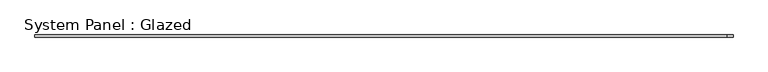
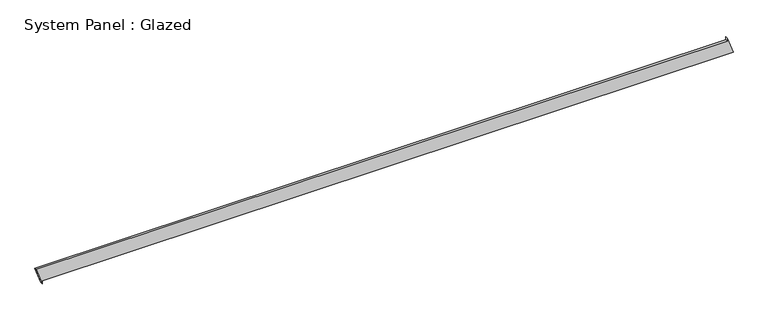
"""IFC4 building model written with IfcOpenShell, lengths in millimetres: plate geometry, System Panel : Glazed."""

import ifcopenshell
import ifcopenshell.guid

model = None  # the IFC model being written
_history = None  # IfcOwnerHistory: only IFC2X3 demands one
_inside = {}  # id of a spatial element -> (the spatial element, [elements in it])
_under = {}  # id of a project, library or spatial element -> (it, [spatial elements below it])
_declared = {}  # id of a project -> (the project, [libraries it declares])
_typed = {}  # id of a type object -> (the type object, [elements of that type])
_made_of = {}  # id of a material, layer set ... -> (it, [elements and type objects made of it])


def new_model(schema):
    """Start an empty IFC model of exactly this schema.

    Asked for "IFC4X3", IfcOpenShell would pick the latest addendum, in which some entities
    have other attributes; the version numbers below select the first issue.
    IFC2X3 requires an IfcOwnerHistory on every rooted entity: one is made here for all.
    """
    global model, _history
    if schema == "IFC4X3":
        model = ifcopenshell.file(schema_version=(4, 3, 0, 0))
    else:
        model = ifcopenshell.file(schema=schema)
    _inside.clear()
    _under.clear()
    _declared.clear()
    _typed.clear()
    _made_of.clear()
    _history = None
    if model.schema == "IFC2X3":
        org = make("IfcOrganization", Name="unknown")
        user = make(
            "IfcPersonAndOrganization",
            ThePerson=make("IfcPerson", FamilyName="unknown"),
            TheOrganization=org,
        )
        app = make(
            "IfcApplication",
            ApplicationDeveloper=org,
            Version="unknown",
            ApplicationFullName="unknown",
            ApplicationIdentifier="unknown",
        )
        _history = make(
            "IfcOwnerHistory",
            OwningUser=user,
            OwningApplication=app,
            ChangeAction="ADDED",
            CreationDate=0,
        )
    return model


def make(cls, **values):
    """One entity of the class cls with the attributes given. An attribute that is None is left unset."""
    return model.create_entity(
        cls, **{name: value for name, value in values.items() if value is not None}
    )


def rooted(cls, **values):
    """An entity with a GlobalId (a new one), such as an element, a storey or a relation."""
    return make(cls, GlobalId=ifcopenshell.guid.new(), OwnerHistory=_history, **values)


def si_unit(unit_type, name, prefix=None):
    """IfcSIUnit, for example si_unit("LENGTHUNIT", "METRE", prefix="MILLI")."""
    return make("IfcSIUnit", UnitType=unit_type, Prefix=prefix, Name=name)


def assignment(units):
    """IfcUnitAssignment: the units of a project."""
    return None if units is None else make("IfcUnitAssignment", Units=units)


def point(xyz):
    """IfcCartesianPoint."""
    return None if xyz is None else make("IfcCartesianPoint", Coordinates=xyz)


def direction(xyz):
    """IfcDirection."""
    return None if xyz is None else make("IfcDirection", DirectionRatios=xyz)


def frame(location, z_axis=None, x_axis=None):
    """IfcAxis2Placement3D, a coordinate frame: its origin and axes. An axis left out is left unset."""
    return make(
        "IfcAxis2Placement3D",
        Location=point(location),
        Axis=direction(z_axis),
        RefDirection=direction(x_axis),
    )


def origin():
    """The frame at (0, 0, 0) with its axes left unset."""
    return frame((0.0, 0.0, 0.0))


def place(relative_to, where):
    """IfcLocalPlacement: puts the frame where relative to a parent placement (None: the world)."""
    return make(
        "IfcLocalPlacement", PlacementRelTo=relative_to, RelativePlacement=where
    )


def context(
    kind, dimensions, precision=None, world=None, true_north=None, identifier=None
):
    """IfcGeometricRepresentationContext, for example the 3D "Model" context."""
    return make(
        "IfcGeometricRepresentationContext",
        ContextIdentifier=identifier,
        ContextType=kind,
        CoordinateSpaceDimension=dimensions,
        Precision=precision,
        WorldCoordinateSystem=world,
        TrueNorth=true_north,
    )


def project(units=None, contexts=None):
    """IfcProject with its units and contexts."""
    return rooted(
        "IfcProject",
        Name="project",
        RepresentationContexts=contexts,
        UnitsInContext=assignment(units),
    )


def spatial(cls, under=None, at=None, **own):
    """A site, building, storey or space (cls), placed at a placement, below another one or the project."""
    s = rooted(cls, ObjectPlacement=at, **own)
    if under is not None:
        _under.setdefault(under.id(), (under, []))[1].append(s)
    return s


def polyline(points):
    """IfcPolyline through the points."""
    return make("IfcPolyline", Points=[point(p) for p in points])


def outline(outer, holes=None, kind="AREA"):
    """IfcArbitraryClosedProfileDef: a profile drawn as a closed curve; with holes, ...WithVoids."""
    if holes is None:
        return make("IfcArbitraryClosedProfileDef", ProfileType=kind, OuterCurve=outer)
    return make(
        "IfcArbitraryProfileDefWithVoids",
        ProfileType=kind,
        OuterCurve=outer,
        InnerCurves=holes,
    )


def extrude(swept, where, along, depth):
    """IfcExtrudedAreaSolid: the profile swept, set in the frame where, extruded along a direction by depth."""
    return make(
        "IfcExtrudedAreaSolid",
        SweptArea=swept,
        Position=where,
        ExtrudedDirection=direction(along),
        Depth=depth,
    )


def shape(context_of_items, identifier, shape_type, items):
    """IfcShapeRepresentation: the items that make up one representation, for example the "Body"."""
    return make(
        "IfcShapeRepresentation",
        ContextOfItems=context_of_items,
        RepresentationIdentifier=identifier,
        RepresentationType=shape_type,
        Items=items,
    )


def source(mapping_origin, context_of_items, identifier, shape_type, items):
    """IfcRepresentationMap: a shape defined once, which mapped items show again and again."""
    return make(
        "IfcRepresentationMap",
        MappingOrigin=mapping_origin,
        MappedRepresentation=shape(context_of_items, identifier, shape_type, items),
    )


def transform(
    local_origin,
    x_axis=None,
    y_axis=None,
    z_axis=None,
    scale=None,
    scale2=None,
    scale3=None,
    uniform=True,
):
    """IfcCartesianTransformationOperator3D, or its non-uniform kind. x_axis, y_axis, z_axis: its Axis1, 2, 3."""
    if uniform:
        return make(
            "IfcCartesianTransformationOperator3D",
            Axis1=direction(x_axis),
            Axis2=direction(y_axis),
            LocalOrigin=point(local_origin),
            Scale=scale,
            Axis3=direction(z_axis),
        )
    return make(
        "IfcCartesianTransformationOperator3DnonUniform",
        Axis1=direction(x_axis),
        Axis2=direction(y_axis),
        LocalOrigin=point(local_origin),
        Scale=scale,
        Axis3=direction(z_axis),
        Scale2=scale2,
        Scale3=scale3,
    )


def mapped(mapping_source, mapping_target):
    """IfcMappedItem: shows the shape of a source again, moved by a transform."""
    return make(
        "IfcMappedItem", MappingSource=mapping_source, MappingTarget=mapping_target
    )


def made_of(thing, what):
    """Note that an element or type object is made of a material, layer set ...; save() writes the relation."""
    if what is not None:
        _made_of.setdefault(what.id(), (what, []))[1].append(thing)
    return thing


def element(
    cls,
    number,
    at=None,
    inside=None,
    cuts=None,
    type_object=None,
    material=None,
    context=None,
    identifier="Body",
    shape_type=None,
    held_by="IfcProductDefinitionShape",
    body=None,
    shapes=None,
    **own,
):
    """One element of the class cls, such as IfcWall. Its Tag is "e" and its number.

    at: its placement. inside: the storey or other place that contains it. cuts: it is an
    opening in that element (IfcRelVoidsElement). A single representation is given by context,
    identifier, shape_type and body (its items); several are given by shapes. held_by: the class
    of the entity that holds the representations. save() writes the other relations.
    """
    e = rooted(cls, Tag="e%d" % number, ObjectPlacement=at, **own)
    if body is not None:
        shapes = [shape(context, identifier, shape_type, body)]
    if shapes is not None:
        e.Representation = make(held_by, Representations=shapes)
    if inside is not None:
        _inside.setdefault(inside.id(), (inside, []))[1].append(e)
    if cuts is not None:
        rooted(
            "IfcRelVoidsElement", RelatingBuildingElement=cuts, RelatedOpeningElement=e
        )
    if type_object is not None:
        _typed.setdefault(type_object.id(), (type_object, []))[1].append(e)
    return made_of(e, material)


def aggregate(whole, parts):
    """IfcRelAggregates: a whole, such as a stair, and the parts it consists of."""
    return rooted("IfcRelAggregates", RelatingObject=whole, RelatedObjects=parts)


def save(model, path):
    """Write the relations noted so far, then the file.

    IfcRelAggregates (storeys below a building ...), IfcRelContainedInSpatialStructure (elements
    in a storey), IfcRelDefinesByType, IfcRelAssociatesMaterial and IfcRelDeclares: one each for
    every whole, place, type object, material and project.
    """
    for whole, parts in _under.values():
        aggregate(whole, parts)
    for where, things in _inside.values():
        rooted(
            "IfcRelContainedInSpatialStructure",
            RelatedElements=things,
            RelatingStructure=where,
        )
    for kind, things in _typed.values():
        rooted("IfcRelDefinesByType", RelatedObjects=things, RelatingType=kind)
    for what, things in _made_of.values():
        rooted("IfcRelAssociatesMaterial", RelatedObjects=things, RelatingMaterial=what)
    for by, libraries in _declared.values():
        rooted("IfcRelDeclares", RelatingContext=by, RelatedDefinitions=libraries)
    model.write(path)


def system_panel_glazed_38c3c94b(model_context):
    return source(origin(), model_context, "Body", "SweptSolid", [
        extrude(outline(polyline([(0.0, -3958.8254362), (35.3553391, -3958.8254362), (35.3553391, 4027.6368042), (234.820266, 3959.126507), (199.4649269, 3959.127058), (199.3404739, -4027.6368042), (0.0, -3958.8254362)])), frame((0.0, -49.5, 0.0), z_axis=(0.0, 1.0, 0.0), x_axis=(0.0, 0.0, 1.0)), (0.0, 0.0, 1.0), 25.0),
    ])


if __name__ == "__main__":
    model = new_model("IFC4")
    model_context = context("Model", 3, world=origin())
    ifc_project = project(units=[si_unit("LENGTHUNIT", "METRE", prefix="MILLI")], contexts=[model_context])
    site = spatial("IfcSite", under=ifc_project)
    building = spatial("IfcBuilding", under=site)
    placement = place(None, origin())
    system_panel_glazed_shape = system_panel_glazed_38c3c94b(model_context)
    element("IfcPlate", 1, ObjectType="System Panel : Glazed", at=placement, inside=building, context=model_context, shape_type="MappedRepresentation", body=[
        mapped(system_panel_glazed_shape, transform((0.0, 0.0, 0.0), x_axis=(1.0, 0.0, 0.0), y_axis=(0.0, 1.0, 0.0), z_axis=(0.0, 0.0, 1.0))),
    ])
    save(model, "model.ifc")

# Revit data of these elements
# Element 1 (IfcPlate, "System Panel : Glazed")
#   Materials on its faces: "Glass"
# Materials
#   "Glass": class "Glass", colour RGB 218 227 224, transparency 0.85, Description = "Soda Lime Glass", Cost = 0
